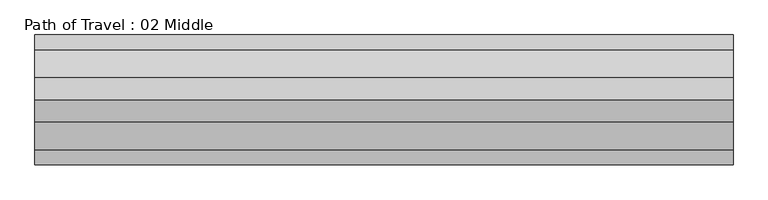
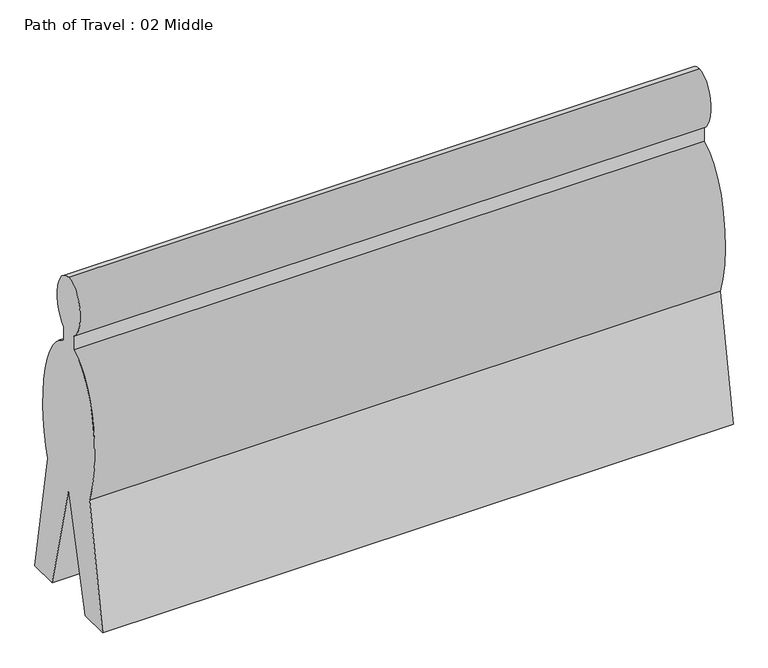
"""IFC4 building model written with IfcOpenShell, lengths in millimetres: proxy geometry, Path of Travel : 02 Middle."""

from ifc_helpers import new_model, si_unit, point, frame, origin, place, context, project, spatial, ellipse_curve, trimmed, source, transform, mapped, element, save
from ifc_brep_helpers import plane_surface, extruded_surface, advanced_brep


def path_of_travel_02_middle_bda6c09b(model_context):
    return source(origin(), model_context, "Body", "AdvancedBrep", [
        advanced_brep(
        [(227.5554837, 0.0, 1727.2), (227.5554837, 42.9018657, 1436.6534209), (227.5554837, 42.9018657, 1363.4763406), (227.5554837, 184.1186263, 643.4144547), (227.5554837, 297.5699544, 0.0), (227.5554837, 145.6574193, 0.0), (227.5554837, 0.0, 584.2), (227.5554837, -145.6574193, 0.0), (227.5554837, -297.5699544, 0.0), (227.5554837, -184.1186263, 643.4144547), (227.5554837, -42.9018657, 1363.4763406), (227.5554837, -42.9018657, 1436.6534209), (3427.9554837, 0.0, 1727.2), (3427.9554837, -42.9018657, 1436.6534209), (3427.9554837, -42.9018657, 1363.4763406), (3427.9554837, -184.1186263, 643.4144547), (3427.9554837, -297.5699544, 0.0), (3427.9554837, -145.6574193, 0.0), (3427.9554837, 0.0, 584.2), (3427.9554837, 145.6574193, 0.0), (3427.9554837, 297.5699544, 0.0), (3427.9554837, 184.1186263, 643.4144547), (3427.9554837, 42.9018657, 1363.4763406), (3427.9554837, 42.9018657, 1436.6534209)],
        [
            (0, 1, ellipse_curve(frame((227.5554837, 0.0, 1574.8), z_axis=(-1.0, 0.0, 0.0), x_axis=(0.0, 0.0, 1.0)), 152.4, 101.6)),
            (1, 2),
            (2, 3, ellipse_curve(frame((227.5554837, 0.0, 914.4), z_axis=(-1.0, 0.0, 0.0), x_axis=(0.0, 0.0, -1.0)), 457.2, 228.6)),
            (3, 4),
            (4, 5),
            (5, 6),
            (6, 7),
            (7, 8),
            (8, 9),
            (9, 10, ellipse_curve(frame((227.5554837, 0.0, 914.4), z_axis=(-1.0, 0.0, 0.0), x_axis=(0.0, 0.0, -1.0)), 457.2, 228.6)),
            (10, 11),
            (11, 0, ellipse_curve(frame((227.5554837, 0.0, 1574.8), z_axis=(-1.0, 0.0, 0.0), x_axis=(0.0, 0.0, 1.0)), 152.4, 101.6)),
            (12, 13, ellipse_curve(frame((3427.9554837, 0.0, 1574.8), z_axis=(1.0, 0.0, 0.0), x_axis=(0.0, 0.0, 1.0)), 152.4, 101.6)),
            (13, 14),
            (14, 15, ellipse_curve(frame((3427.9554837, 0.0, 914.4), z_axis=(1.0, 0.0, 0.0), x_axis=(0.0, 0.0, -1.0)), 457.2, 228.6)),
            (15, 16),
            (16, 17),
            (17, 18),
            (18, 19),
            (19, 20),
            (20, 21),
            (21, 22, ellipse_curve(frame((3427.9554837, 0.0, 914.4), z_axis=(1.0, 0.0, 0.0), x_axis=(0.0, 0.0, -1.0)), 457.2, 228.6)),
            (22, 23),
            (23, 12, ellipse_curve(frame((3427.9554837, 0.0, 1574.8), z_axis=(1.0, 0.0, 0.0), x_axis=(0.0, 0.0, 1.0)), 152.4, 101.6)),
            (0, 12),
            (23, 1),
            (22, 2),
            (21, 3),
            (20, 4),
            (19, 5),
            (18, 6),
            (17, 7),
            (16, 8),
            (15, 9),
            (14, 10),
            (13, 11),
        ],
        [
            plane_surface(frame((227.5554837, 0.0, 0.0), z_axis=(-1.0, 0.0, 0.0), x_axis=(0.0, 0.0, 1.0))),
            plane_surface(frame((3427.9554837, 0.0, 0.0), z_axis=(1.0, 0.0, 0.0), x_axis=(0.0, 0.0, 1.0))),
            extruded_surface(trimmed(ellipse_curve(frame((3427.9554837, 0.0, 1574.8), z_axis=(-1.0, 0.0, 0.0), x_axis=(0.0, 0.0, 1.0)), 152.4, 101.6), [point((3427.9554837, 0.0, 1727.2))], [point((3427.9554837, 42.9018657, 1436.6534209))], True, "CARTESIAN"), (-3200.4, 0.0, 0.0), 3200.4),
            plane_surface(frame((227.5554837, 42.9018657, 1436.6534209), z_axis=(0.0, 1.0, 0.0), x_axis=(1.0, 0.0, 0.0))),
            extruded_surface(trimmed(ellipse_curve(frame((3427.9554837, 0.0, 914.4), z_axis=(-1.0, 0.0, 0.0), x_axis=(0.0, 0.0, -1.0)), 457.2, 228.6), [point((3427.9554837, 42.9018657, 1363.4763406))], [point((3427.9554837, 184.1186263, 643.4144547))], True, "CARTESIAN"), (-3200.4, 0.0, 0.0), 3200.4),
            plane_surface(frame((227.5554837, 184.1186263, 643.4144547), z_axis=(0.0, 0.9848077530122078, 0.17364817766693205), x_axis=(1.0, 0.0, 0.0))),
            plane_surface(frame((227.5554837, 297.5699544, 0.0), z_axis=(0.0, 0.0, -1.0), x_axis=(1.0, 0.0, 0.0))),
            plane_surface(frame((227.5554837, 145.6574193, 0.0), z_axis=(0.0, -0.9702957262760199, -0.2419218955995739), x_axis=(1.0, 0.0, 0.0))),
            plane_surface(frame((227.5554837, 0.0, 584.2), z_axis=(0.0, 0.9702957262759961, -0.24192189559966923), x_axis=(1.0, 0.0, 0.0))),
            plane_surface(frame((227.5554837, -145.6574193, 0.0), z_axis=(0.0, 0.0, -1.0), x_axis=(1.0, 0.0, 0.0))),
            plane_surface(frame((227.5554837, -297.5699544, 0.0), z_axis=(0.0, -0.984807753012208, 0.17364817766693066), x_axis=(1.0, 0.0, 0.0))),
            extruded_surface(trimmed(ellipse_curve(frame((3427.9554837, 0.0, 914.4), z_axis=(-1.0, 0.0, 0.0), x_axis=(0.0, 0.0, -1.0)), 457.2, 228.6), [point((3427.9554837, -184.1186263, 643.4144547))], [point((3427.9554837, -42.9018657, 1363.4763406))], True, "CARTESIAN"), (-3200.4, 0.0, 0.0), 3200.4),
            plane_surface(frame((227.5554837, -42.9018657, 1363.4763406), z_axis=(0.0, -1.0, 0.0), x_axis=(1.0, 0.0, 0.0))),
            extruded_surface(trimmed(ellipse_curve(frame((3427.9554837, 0.0, 1574.8), z_axis=(-1.0, 0.0, 0.0), x_axis=(0.0, 0.0, 1.0)), 152.4, 101.6), [point((3427.9554837, -42.9018657, 1436.6534209))], [point((3427.9554837, 0.0, 1727.2))], True, "CARTESIAN"), (-3200.4, 0.0, 0.0), 3200.4),
        ],
        [
            (0, [[1, 2, 3, 4, 5, 6, 7, 8, 9, 10, 11, 12]]),
            (1, [[13, 14, 15, 16, 17, 18, 19, 20, 21, 22, 23, 24]]),
            (2, [[-1, 25, -24, 26]]),
            (3, [[-2, -26, -23, 27]]),
            (4, [[-3, -27, -22, 28]]),
            (5, [[-4, -28, -21, 29]]),
            (6, [[-5, -29, -20, 30]]),
            (7, [[-6, -30, -19, 31]]),
            (8, [[-7, -31, -18, 32]]),
            (9, [[-8, -32, -17, 33]]),
            (10, [[-9, -33, -16, 34]]),
            (11, [[-10, -34, -15, 35]]),
            (12, [[-11, -35, -14, 36]]),
            (13, [[-12, -36, -13, -25]]),
        ],
    ),
    ])


if __name__ == "__main__":
    model = new_model("IFC4")
    model_context = context("Model", 3, world=origin())
    ifc_project = project(units=[si_unit("LENGTHUNIT", "METRE", prefix="MILLI")], contexts=[model_context])
    site = spatial("IfcSite", under=ifc_project)
    building = spatial("IfcBuilding", under=site)
    placement = place(None, origin())
    path_of_travel_02_middle_shape = path_of_travel_02_middle_bda6c09b(model_context)
    element("IfcBuildingElementProxy", 1, Name="Path of Travel : 02 Middle", ObjectType="Path of Travel : 02 Middle", at=placement, inside=building, context=model_context, shape_type="MappedRepresentation", body=[
        mapped(path_of_travel_02_middle_shape, transform((0.0, 0.0, 0.0), x_axis=(1.0, 0.0, 0.0), y_axis=(0.0, 1.0, 0.0), z_axis=(0.0, 0.0, 1.0))),
    ])
    save(model, "model.ifc")

# Revit data of these elements
# Type "Path of Travel : 02 Middle"
#   Path of Egress [instance default] = 4' - 0"
#   built-in parameter 1001306 [instance default] = 4 (stored number, unit not read)
#   Dot at Start = no
#   Arrow in Middle = yes
#   Arrow at End = no
#   Egress Path = none
# Element 1 (IfcBuildingElementProxy, "Path of Travel : 02 Middle")
#   Path of Egress = 10' - 6"
#   built-in parameter 1001306 = 10.5 (stored number, unit not read)
#   Materials on its faces: "Egress Path Solid"
# Materials
#   "Egress Path Solid": class "Unassigned", colour RGB 255 128 64, transparency 0.75, Comments = "Rendering appearance not upgraded "
